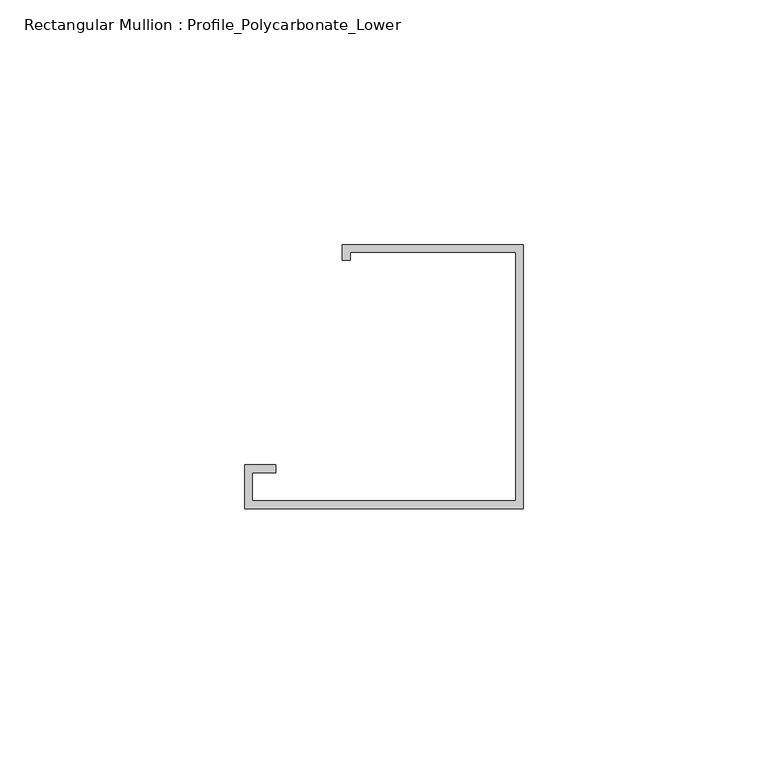
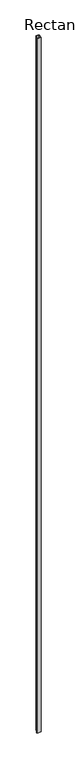
"""IFC4 building model written with IfcOpenShell, lengths in millimetres: member geometry, Rectangular Mullion : Profile_Polycarbonate_Lower."""

from ifc_helpers import new_model, si_unit, frame, origin, place, context, project, spatial, polyline, outline, extrude, source, transform, mapped, element, save


def rectangular_mullion_profile_polycarbonate_lower_6a1ad31b(model_context):
    return source(origin(), model_context, "Body", "SweptSolid", [
        extrude(outline(polyline([(0.0, -28.984575), (-56.9976, -28.984575), (-56.9976, -19.992975), (-50.6476, -19.992975), (-50.6476, -21.580475), (-55.4101, -21.580475), (-55.4101, -27.397075), (-1.5875, -27.397075), (-1.5875, 23.428325), (-35.3949, 23.428325), (-35.3949, 21.840825), (-36.9824, 21.840825), (-36.9824, 25.015825), (0.0, 25.015825), (0.0, -28.984575)])), frame((0.0, 0.0, -9969.6524), z_axis=(0.0, 0.0, 1.0), x_axis=(1.0, 0.0, 0.0)), (0.0, 0.0, 1.0), 9969.6524),
    ])


if __name__ == "__main__":
    model = new_model("IFC4")
    model_context = context("Model", 3, world=origin())
    ifc_project = project(units=[si_unit("LENGTHUNIT", "METRE", prefix="MILLI")], contexts=[model_context])
    site = spatial("IfcSite", under=ifc_project)
    building = spatial("IfcBuilding", under=site)
    placement = place(None, origin())
    rectangular_mullion_profile_polycarbonate_lower_shape = rectangular_mullion_profile_polycarbonate_lower_6a1ad31b(model_context)
    element("IfcMember", 1, ObjectType="Rectangular Mullion : Profile_Polycarbonate_Lower", at=placement, inside=building, context=model_context, shape_type="MappedRepresentation", body=[
        mapped(rectangular_mullion_profile_polycarbonate_lower_shape, transform((0.0, 0.0, 0.0), x_axis=(1.0, 0.0, 0.0), y_axis=(0.0, 1.0, 0.0), z_axis=(0.0, 0.0, 1.0))),
    ])
    save(model, "model.ifc")

# Revit data of these elements
# Type "Rectangular Mullion : Profile_Polycarbonate_Lower"
#   built-in parameter 1007322 = 0.177167 (stored number, unit not read)
#   built-in parameter 1007321 = 0 (stored number, unit not read)
#   built-in parameter 1007320 = 0.00520833 (stored number, unit not read)
